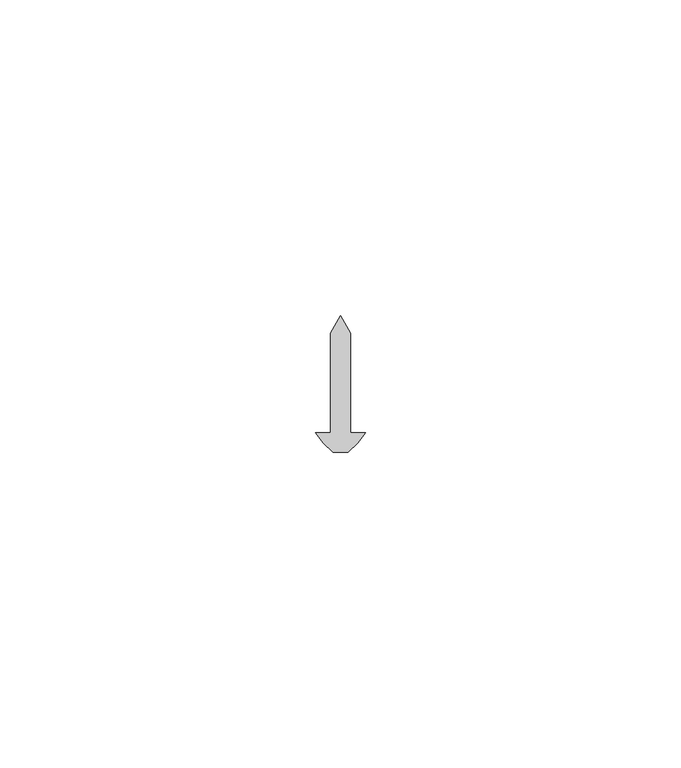
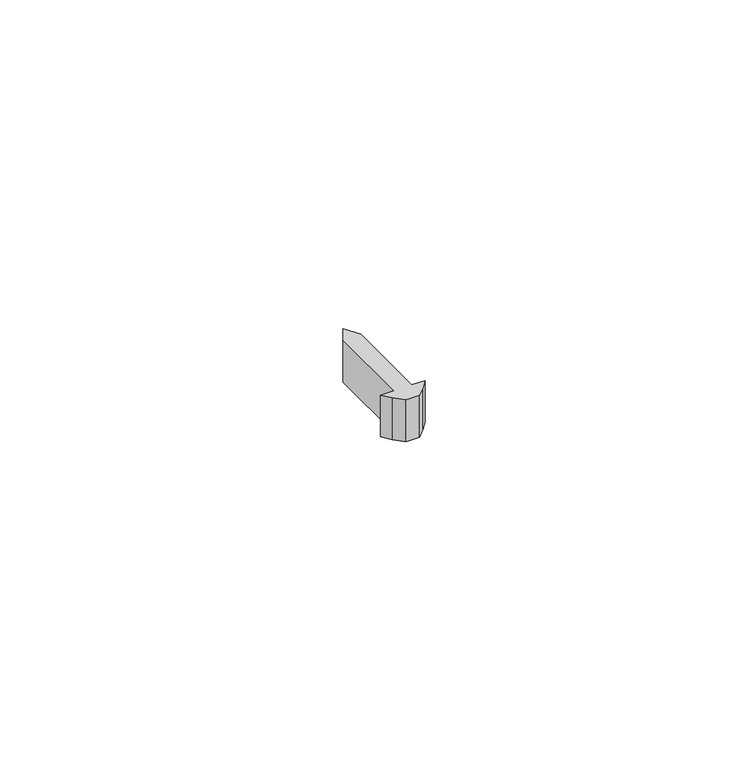
"""IFC4 building model written with IfcOpenShell, lengths in millimetres: proxy geometry, Generic Models 7:Generic Models 1:3:Generic Models 1:3 : Generic Models 7:Generic Models 1:305549:3:Generic Models 1:3:Generic Models 1:3 : Generic Models 7:Generic Models 1:305549:3 : Generic Models 7:Generic Models 1:3:Generic Models 1:3 : Generic Models 7:Generic Models 1:305549:301244:53 : Generic Models 7:Generic Models 1:3:Generic Models 1:3 : Generic Models 7:Generic Models 1:305549:3:Generic Models 1:3:Generic Models 1:3 : Generic Models 7:Generic Models 1:305549:3 : Generic Models 7:Generic Models 1:3:Generic Models 1:3 : Generic Models 7:Generic Models 1:305549:301244:308848."""

import ifcopenshell
import ifcopenshell.guid

model = None  # the IFC model being written
_history = None  # IfcOwnerHistory: only IFC2X3 demands one
_inside = {}  # id of a spatial element -> (the spatial element, [elements in it])
_under = {}  # id of a project, library or spatial element -> (it, [spatial elements below it])
_declared = {}  # id of a project -> (the project, [libraries it declares])
_typed = {}  # id of a type object -> (the type object, [elements of that type])
_made_of = {}  # id of a material, layer set ... -> (it, [elements and type objects made of it])


def new_model(schema):
    """Start an empty IFC model of exactly this schema.

    Asked for "IFC4X3", IfcOpenShell would pick the latest addendum, in which some entities
    have other attributes; the version numbers below select the first issue.
    IFC2X3 requires an IfcOwnerHistory on every rooted entity: one is made here for all.
    """
    global model, _history
    if schema == "IFC4X3":
        model = ifcopenshell.file(schema_version=(4, 3, 0, 0))
    else:
        model = ifcopenshell.file(schema=schema)
    _inside.clear()
    _under.clear()
    _declared.clear()
    _typed.clear()
    _made_of.clear()
    _history = None
    if model.schema == "IFC2X3":
        org = make("IfcOrganization", Name="unknown")
        user = make(
            "IfcPersonAndOrganization",
            ThePerson=make("IfcPerson", FamilyName="unknown"),
            TheOrganization=org,
        )
        app = make(
            "IfcApplication",
            ApplicationDeveloper=org,
            Version="unknown",
            ApplicationFullName="unknown",
            ApplicationIdentifier="unknown",
        )
        _history = make(
            "IfcOwnerHistory",
            OwningUser=user,
            OwningApplication=app,
            ChangeAction="ADDED",
            CreationDate=0,
        )
    return model


def make(cls, **values):
    """One entity of the class cls with the attributes given. An attribute that is None is left unset."""
    return model.create_entity(
        cls, **{name: value for name, value in values.items() if value is not None}
    )


def rooted(cls, **values):
    """An entity with a GlobalId (a new one), such as an element, a storey or a relation."""
    return make(cls, GlobalId=ifcopenshell.guid.new(), OwnerHistory=_history, **values)


def si_unit(unit_type, name, prefix=None):
    """IfcSIUnit, for example si_unit("LENGTHUNIT", "METRE", prefix="MILLI")."""
    return make("IfcSIUnit", UnitType=unit_type, Prefix=prefix, Name=name)


def assignment(units):
    """IfcUnitAssignment: the units of a project."""
    return None if units is None else make("IfcUnitAssignment", Units=units)


def point(xyz):
    """IfcCartesianPoint."""
    return None if xyz is None else make("IfcCartesianPoint", Coordinates=xyz)


def direction(xyz):
    """IfcDirection."""
    return None if xyz is None else make("IfcDirection", DirectionRatios=xyz)


def frame(location, z_axis=None, x_axis=None):
    """IfcAxis2Placement3D, a coordinate frame: its origin and axes. An axis left out is left unset."""
    return make(
        "IfcAxis2Placement3D",
        Location=point(location),
        Axis=direction(z_axis),
        RefDirection=direction(x_axis),
    )


def origin():
    """The frame at (0, 0, 0) with its axes left unset."""
    return frame((0.0, 0.0, 0.0))


def place(relative_to, where):
    """IfcLocalPlacement: puts the frame where relative to a parent placement (None: the world)."""
    return make(
        "IfcLocalPlacement", PlacementRelTo=relative_to, RelativePlacement=where
    )


def context(
    kind, dimensions, precision=None, world=None, true_north=None, identifier=None
):
    """IfcGeometricRepresentationContext, for example the 3D "Model" context."""
    return make(
        "IfcGeometricRepresentationContext",
        ContextIdentifier=identifier,
        ContextType=kind,
        CoordinateSpaceDimension=dimensions,
        Precision=precision,
        WorldCoordinateSystem=world,
        TrueNorth=true_north,
    )


def project(units=None, contexts=None):
    """IfcProject with its units and contexts."""
    return rooted(
        "IfcProject",
        Name="project",
        RepresentationContexts=contexts,
        UnitsInContext=assignment(units),
    )


def spatial(cls, under=None, at=None, **own):
    """A site, building, storey or space (cls), placed at a placement, below another one or the project."""
    s = rooted(cls, ObjectPlacement=at, **own)
    if under is not None:
        _under.setdefault(under.id(), (under, []))[1].append(s)
    return s


def polyline(points):
    """IfcPolyline through the points."""
    return make("IfcPolyline", Points=[point(p) for p in points])


def outline(outer, holes=None, kind="AREA"):
    """IfcArbitraryClosedProfileDef: a profile drawn as a closed curve; with holes, ...WithVoids."""
    if holes is None:
        return make("IfcArbitraryClosedProfileDef", ProfileType=kind, OuterCurve=outer)
    return make(
        "IfcArbitraryProfileDefWithVoids",
        ProfileType=kind,
        OuterCurve=outer,
        InnerCurves=holes,
    )


def extrude(swept, where, along, depth):
    """IfcExtrudedAreaSolid: the profile swept, set in the frame where, extruded along a direction by depth."""
    return make(
        "IfcExtrudedAreaSolid",
        SweptArea=swept,
        Position=where,
        ExtrudedDirection=direction(along),
        Depth=depth,
    )


def shape(context_of_items, identifier, shape_type, items):
    """IfcShapeRepresentation: the items that make up one representation, for example the "Body"."""
    return make(
        "IfcShapeRepresentation",
        ContextOfItems=context_of_items,
        RepresentationIdentifier=identifier,
        RepresentationType=shape_type,
        Items=items,
    )


def source(mapping_origin, context_of_items, identifier, shape_type, items):
    """IfcRepresentationMap: a shape defined once, which mapped items show again and again."""
    return make(
        "IfcRepresentationMap",
        MappingOrigin=mapping_origin,
        MappedRepresentation=shape(context_of_items, identifier, shape_type, items),
    )


def transform(
    local_origin,
    x_axis=None,
    y_axis=None,
    z_axis=None,
    scale=None,
    scale2=None,
    scale3=None,
    uniform=True,
):
    """IfcCartesianTransformationOperator3D, or its non-uniform kind. x_axis, y_axis, z_axis: its Axis1, 2, 3."""
    if uniform:
        return make(
            "IfcCartesianTransformationOperator3D",
            Axis1=direction(x_axis),
            Axis2=direction(y_axis),
            LocalOrigin=point(local_origin),
            Scale=scale,
            Axis3=direction(z_axis),
        )
    return make(
        "IfcCartesianTransformationOperator3DnonUniform",
        Axis1=direction(x_axis),
        Axis2=direction(y_axis),
        LocalOrigin=point(local_origin),
        Scale=scale,
        Axis3=direction(z_axis),
        Scale2=scale2,
        Scale3=scale3,
    )


def mapped(mapping_source, mapping_target):
    """IfcMappedItem: shows the shape of a source again, moved by a transform."""
    return make(
        "IfcMappedItem", MappingSource=mapping_source, MappingTarget=mapping_target
    )


def made_of(thing, what):
    """Note that an element or type object is made of a material, layer set ...; save() writes the relation."""
    if what is not None:
        _made_of.setdefault(what.id(), (what, []))[1].append(thing)
    return thing


def element(
    cls,
    number,
    at=None,
    inside=None,
    cuts=None,
    type_object=None,
    material=None,
    context=None,
    identifier="Body",
    shape_type=None,
    held_by="IfcProductDefinitionShape",
    body=None,
    shapes=None,
    **own,
):
    """One element of the class cls, such as IfcWall. Its Tag is "e" and its number.

    at: its placement. inside: the storey or other place that contains it. cuts: it is an
    opening in that element (IfcRelVoidsElement). A single representation is given by context,
    identifier, shape_type and body (its items); several are given by shapes. held_by: the class
    of the entity that holds the representations. save() writes the other relations.
    """
    e = rooted(cls, Tag="e%d" % number, ObjectPlacement=at, **own)
    if body is not None:
        shapes = [shape(context, identifier, shape_type, body)]
    if shapes is not None:
        e.Representation = make(held_by, Representations=shapes)
    if inside is not None:
        _inside.setdefault(inside.id(), (inside, []))[1].append(e)
    if cuts is not None:
        rooted(
            "IfcRelVoidsElement", RelatingBuildingElement=cuts, RelatedOpeningElement=e
        )
    if type_object is not None:
        _typed.setdefault(type_object.id(), (type_object, []))[1].append(e)
    return made_of(e, material)


def aggregate(whole, parts):
    """IfcRelAggregates: a whole, such as a stair, and the parts it consists of."""
    return rooted("IfcRelAggregates", RelatingObject=whole, RelatedObjects=parts)


def save(model, path):
    """Write the relations noted so far, then the file.

    IfcRelAggregates (storeys below a building ...), IfcRelContainedInSpatialStructure (elements
    in a storey), IfcRelDefinesByType, IfcRelAssociatesMaterial and IfcRelDeclares: one each for
    every whole, place, type object, material and project.
    """
    for whole, parts in _under.values():
        aggregate(whole, parts)
    for where, things in _inside.values():
        rooted(
            "IfcRelContainedInSpatialStructure",
            RelatedElements=things,
            RelatingStructure=where,
        )
    for kind, things in _typed.values():
        rooted("IfcRelDefinesByType", RelatedObjects=things, RelatingType=kind)
    for what, things in _made_of.values():
        rooted("IfcRelAssociatesMaterial", RelatedObjects=things, RelatingMaterial=what)
    for by, libraries in _declared.values():
        rooted("IfcRelDeclares", RelatingContext=by, RelatedDefinitions=libraries)
    model.write(path)


def generic_models_2602704b(model_context):
    return source(origin(), model_context, "Body", "SweptSolid", [
        extrude(outline(polyline([(579001.3242239, -579084.8288841), (579003.7054739, -579084.8288841), (579002.4872784, -579086.3559421), (579000.9353882, -579087.9078323), (578998.5380597, -579087.9078323), (578996.9861695, -579086.3559421), (578995.7679739, -579084.8288841), (578998.1492239, -579084.8288841), (578998.1492239, -579069.0196286), (578999.7367239, -579066.2699979), (579001.3242239, -579069.0196286), (579001.3242239, -579084.8288841)])), frame((0.0, 0.0, 4907.75625), z_axis=(0.0, 0.0, 1.0), x_axis=(1.0, 0.0, 0.0)), (0.0, 0.0, 1.0), 7.9375),
    ])


if __name__ == "__main__":
    model = new_model("IFC4")
    model_context = context("Model", 3, world=origin())
    ifc_project = project(units=[si_unit("LENGTHUNIT", "METRE", prefix="MILLI")], contexts=[model_context])
    site = spatial("IfcSite", under=ifc_project)
    building = spatial("IfcBuilding", under=site)
    placement = place(None, origin())
    generic_models_shape = generic_models_2602704b(model_context)
    element("IfcBuildingElementProxy", 1, Name="Generic Models 7:Generic Models 1:3:Generic Models 1:3 : Generic Models 7:Generic Models 1:305549:3:Generic Models 1:3:Generic Models 1:3 : Generic Models 7:Generic Models 1:305549:3 : Generic Models 7:Generic Models 1:3:Generic Models 1:3 : Generic Models 7:Generic Models 1:305549:301244:53 : Generic Models 7:Generic Models 1:3:Generic Models 1:3 : Generic Models 7:Generic Models 1:305549:3:Generic Models 1:3:Generic Models 1:3 : Generic Models 7:Generic Models 1:305549:3 : Generic Models 7:Generic Models 1:3:Generic Models 1:3 : Generic Models 7:Generic Models 1:305549:301244:308848", ObjectType="Generic Models 7:Generic Models 1:3:Generic Models 1:3 : Generic Models 7:Generic Models 1:305549:3:Generic Models 1:3:Generic Models 1:3 : Generic Models 7:Generic Models 1:305549:3 : Generic Models 7:Generic Models 1:3:Generic Models 1:3 : Generic Models 7:Generic Models 1:305549:301244:53 : Generic Models 7:Generic Models 1:3:Generic Models 1:3 : Generic Models 7:Generic Models 1:305549:3:Generic Models 1:3:Generic Models 1:3 : Generic Models 7:Generic Models 1:305549:3 : Generic Models 7:Generic Models 1:3:Generic Models 1:3 : Generic Models 7:Generic Models 1:305549:301244:308848", at=placement, inside=building, context=model_context, shape_type="MappedRepresentation", body=[
        mapped(generic_models_shape, transform((0.0, 0.0, 0.0), x_axis=(1.0, 0.0, 0.0), y_axis=(0.0, 1.0, 0.0), z_axis=(0.0, 0.0, 1.0))),
    ])
    save(model, "model.ifc")

# Revit data of these elements
# Type "Generic Models 7:Generic Models 1:3:Generic Models 1:3 : Generic Models 7:Generic Models 1:305549:3:Generic Models 1:3:Generic Models 1:3 : Generic Models 7:Generic Models 1:305549:3 : Generic Models 7:Generic Models 1:3:Generic Models 1:3 : Generic Models 7:Generic Models 1:305549:301244:53 : Generic Models 7:Generic Models 1:3:Generic Models 1:3 : Generic Models 7:Generic Models 1:305549:3:Generic Models 1:3:Generic Models 1:3 : Generic Models 7:Generic Models 1:305549:3 : Generic Models 7:Generic Models 1:3:Generic Models 1:3 : Generic Models 7:Generic Models 1:305549:301244:308848"
#   NameOverride = "Generic Models 7:Generic Models 1:3:Generic Models 1:3 : Generic Models 7:Generic Models 1:305549:3:Generic Models 1:3:Generic Models 1:3 : Generic Models 7:Generic Models 1:305549:3 : Generic Models 7:Generic Models 1:3:Generic Models 1:3 : Generic Models 7:Generic Models 1:305549:301244:308848"
#   ObjectTypeOverride = "Generic Models 1:3:Generic Models 1:3 : Generic Models 7:Generic Models 1:305549:3 : Generic Models 7:Generic Models 1:3:Generic Models 1:3 : Generic Models 7:Generic Models 1:305549:301244"
#   Reference = "Generic Models 1"
#   Tag = "308848"
# Element 1 (IfcBuildingElementProxy, "Generic Models 7:Generic Models 1:3:Generic Models 1:3 : Generic Models 7:Generic Models 1:305549:3:Generic Models 1:3:Generic Models 1:3 : Generic Models 7:Generic Models 1:305549:3 : Generic Models 7:Generic Models 1:3:Generic Models 1:3 : Generic Models 7:Generic Models 1:305549:301244:53 : Generic Models 7:Generic Models 1:3:Generic Models 1:3 : Generic Models 7:Generic Models 1:305549:3:Generic Models 1:3:Generic Models 1:3 : Generic Models 7:Generic Models 1:305549:3 : Generic Models 7:Generic Models 1:3:Generic Models 1:3 : Generic Models 7:Generic Models 1:305549:301244:308848")
#   Materials on its faces: "FASTENERS (T.B.D)"
# Materials
#   "FASTENERS (T.B.D)": class "Generic", colour RGB 120 120 120, transparency 0, Cost = 0
